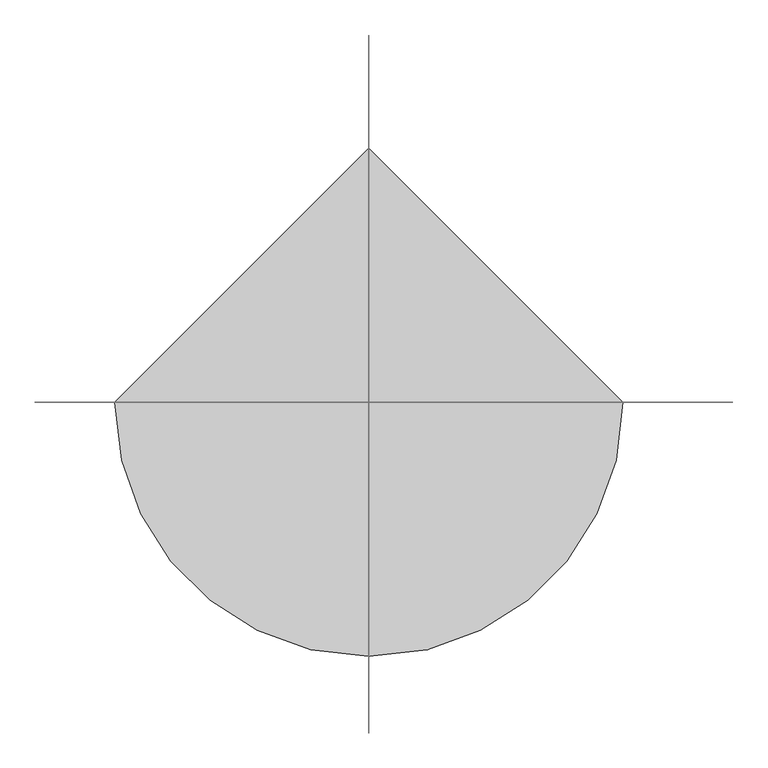
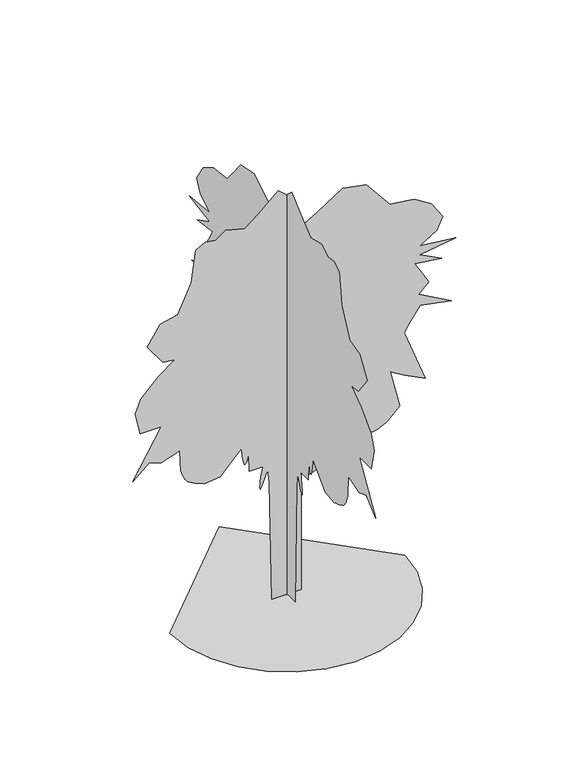
"""IFC4 building model written with IfcOpenShell, lengths in millimetres: proxy geometry, windmill palm 26123 : windmill palm 26123."""

from ifc_helpers import new_model, si_unit, origin, place, context, project, spatial, triangles, source, transform, mapped, element, save


def entourage_d7a905c7(model_context):
    return source(origin(), model_context, "Body", "Tessellation", [
        triangles([(-0.2241189, -80.6803134, 0.0560704), (-0.2241181, -93.4507094, 708.3955685), (-0.2241176, -102.9729479, 784.5729681), (-0.2241171, -112.4304103, 759.6428038), (-0.2241163, -121.4992608, 736.1299221), (-0.2241158, -129.7908604, 715.4466642), (-0.2241156, -136.916343, 699.0127836), (-0.2241151, -142.4870876, 688.2406214), (-0.2241151, -146.1147278, 684.5474602), (-0.2241148, -147.4101338, 689.3505827), (-0.2241148, -146.9475984, 700.5392893), (-0.2241151, -145.6519381, 714.7252693), (-0.2241151, -143.662352, 731.4105881), (-0.2241153, -141.1175219, 750.0923693), (-0.2241156, -138.1563745, 770.2752216), (-0.2241156, -134.9173553, 791.458885), (-0.2241158, -131.5396545, 813.1404104), (-0.2241113, -207.7180624, 813.1404104), (-0.224111, -210.8920511, 914.7103008), (-0.2241108, -214.9636775, 900.580204), (-0.2241105, -218.9799477, 887.367057), (-0.2241105, -222.88496, 875.9827955), (-0.2241103, -226.6235945, 867.3493109), (-0.22411, -230.1402221, 862.3810095), (-0.2241097, -233.3789961, 861.9923704), (-0.2241095, -236.2847599, 867.1003435), (-0.2241095, -238.9129061, 876.4653969), (-0.2241092, -241.3744383, 887.9944897), (-0.2241092, -243.6972616, 901.3295042), (-0.224109, -245.9088635, 916.1097794), (-0.224109, -248.0373855, 931.9696398), (-0.2241087, -250.1102786, 948.5533659), (-0.2241087, -252.1552483, 965.4977531), (-0.2241016, -372.7715778, 838.5329012), (-0.2240963, -461.6464946, 829.010372), (-0.224095, -479.2563572, 835.8125004), (-0.224094, -496.4217339, 842.6147015), (-0.2240932, -512.6981023, 849.4168299), (-0.2240922, -527.64352, 856.2164148), (-0.2240914, -540.8134646, 863.0185432), (-0.2240907, -551.7608706, 869.8206717), (-0.2240902, -560.0413244, 876.6228727), (-0.2240899, -566.4726179, 884.1641275), (-0.2240897, -572.238436, 893.0389492), (-0.2240892, -577.4480018, 903.0236595), (-0.2240889, -582.2155887, 913.8974871), (-0.2240887, -586.6479126, 925.4367537), (-0.2240884, -590.8567037, 937.4204699), (-0.2240881, -594.9562717, 949.6252481), (-0.2240879, -601.3062839, 1073.4150759), (-0.2240815, -706.0511621, 1038.5001286), (-0.2240775, -775.8810568, 1063.8925467), (-0.2240719, -867.928418, 981.3677147), (-0.2240815, -706.0511621, 1254.3398609), (-0.2240744, -826.6659657, 1254.3398609), (-0.2240727, -855.233408, 1381.3021694), (-0.2240747, -823.4909414, 1460.6545933), (-0.2240805, -725.0961479, 1562.224411), (-0.2240861, -629.8712191, 1632.0567764), (-0.2240821, -699.7011137, 1641.5768349), (-0.224077, -785.4035133, 1759.0190849), (-0.2240813, -712.3985945, 1873.2865288), (-0.2240871, -614.0012575, 1895.5039227), (-0.2240917, -537.8238579, 2060.5586735), (-0.2240932, -512.4314034, 2247.8284927), (-0.2240963, -458.4714704, 2276.3959351), (-0.2240998, -398.1640686, 2266.8734058), (-0.2241034, -341.0291113, 2308.1358582), (-0.2241097, -233.1107712, 2279.5708866), (-0.2241143, -156.9326267, 2339.8783974), (-0.2241212, -42.6652782, 2438.2757343), (-0.2241265, 46.2093524, 2358.9233105), (-0.2241265, 46.2093524, 2263.6984543), (-0.2241298, 103.3427746, 2190.6960789), (-0.2241346, 182.6954255, 2235.1334827), (-0.224143, 322.3549604, 2327.1809166), (-0.2241509, 455.6672811, 2301.7884258), (-0.2241557, 538.1921494, 2200.2186081), (-0.2241588, 588.979638, 2136.7361458), (-0.2241672, 728.6394636, 2117.6910873), (-0.224173, 827.0368006, 2057.3837219), (-0.2241768, 890.5167194, 1958.986385), (-0.2241748, 855.6017721, 1889.1564903), (-0.2241689, 760.3793867, 1828.8489796), (-0.2241811, 963.5216383, 1806.6315857), (-0.2241689, 760.3793867, 1774.8890465), (-0.2241763, 884.1692144, 1711.4067295), (-0.2241674, 731.8118717, 1730.4516426), (-0.224172, 811.1642956, 1593.9668049), (-0.2241687, 754.0318817, 1540.0068718), (-0.2241796, 938.1291475, 1435.2621025), (-0.2241692, 763.5544109, 1470.1769772), (-0.2241654, 700.0719486, 1384.477121), (-0.2241636, 671.5045063, 1336.8647655), (-0.224171, 792.1193098, 1022.630167), (-0.2241639, 674.6795305, 1079.7650517), (-0.224159, 592.1520824, 1130.5500332), (-0.2241621, 646.1120155, 908.3627958), (-0.2241583, 579.4571451, 841.7079254), (-0.2241575, 566.5462689, 834.2758209), (-0.2241567, 553.721761, 827.1511105), (-0.224156, 541.0623593, 820.6359558), (-0.2241552, 528.6518887, 815.0378237), (-0.2241544, 516.5766809, 810.6613466), (-0.2241537, 504.9155105, 807.8089771), (-0.2241532, 493.7572526, 806.7929054), (-0.2241524, 482.6879065, 807.6260668), (-0.2241519, 471.2883479, 809.9577559), (-0.2241511, 459.6093733, 813.5392233), (-0.2241504, 447.7094456, 818.1188129), (-0.2241496, 435.6418682, 823.4503189), (-0.2241489, 423.4625244, 829.2796143), (-0.2241481, 411.2298409, 835.357877), (-0.2241481, 407.7779803, 839.4116993), (-0.2241478, 404.0213056, 843.2979446), (-0.2241476, 399.6524952, 846.8514341), (-0.2241471, 394.3692784, 849.9070616), (-0.2241468, 387.8643339, 852.2946339), (-0.2241463, 379.8302676, 853.8491175), (-0.2241458, 369.9674249, 854.4028627), (-0.224145, 357.1403735, 855.883659), (-0.224144, 340.8157522, 860.0289728), (-0.2241428, 321.5777186, 866.3967527), (-0.2241415, 300.0079778, 874.5400057), (-0.2241402, 276.6881621, 884.0168255), (-0.2241387, 252.2014664, 894.3800737), (-0.2241372, 227.1326114, 905.1877716), (-0.2241349, 185.8694142, 857.577887), (-0.2241349, 185.8694142, 778.2254631), (-0.2241362, 208.0876256, 702.0480635), (-0.2241316, 131.9097354, 676.6556454), (-0.2241288, 87.4725496, 800.4429296), (-0.2241293, 88.096376, 0.0), (-666.8181644, -2.5e-06, 0.2128606), (-649.2007078, -152.6793797, 0.2128611), (-599.0329851, -292.8908795, 0.2128626), (-520.3257617, -416.61723, 0.2128649), (-417.1023385, -519.8431603, 0.2128679), (-293.3760243, -598.5478403, 0.2128717), (-153.1642702, -648.715563, 0.2128758), (-0.4850755, -666.3330196, 0.2128804), (152.1942349, -648.715563, 0.2128849), (292.4057347, -598.5478403, 0.212889), (416.1320852, -519.8406169, 0.2128928), (519.3580155, -416.61723, 0.2128959), (598.0626955, -292.8908795, 0.2128981), (648.2304182, -152.6791254, 0.2128997), (665.8478748, 5.82e-05, 0.2129002), (-0.4851924, 666.3330196, 0.2128804), (-89.341994, 0.0001455, 0.1894216), (-102.11239, 0.0001057, 708.5276825), (-111.6346285, 9.96e-05, 784.7075529), (-121.0920909, 0.0001025, 759.7773886), (-130.1609414, 0.0001023, 736.2619635), (-138.4522867, 0.0001051, 715.581249), (-145.5777693, 0.000105, 699.144825), (-151.1487682, 0.0001048, 688.3726627), (-154.7761631, 0.0001075, 684.682045), (-156.0718144, 0.0001043, 689.4852402), (-155.6090338, 0.0001041, 700.6714033), (-154.3136187, 0.0001037, 714.8573833), (-152.3240326, 0.0001034, 731.5426294), (-149.7792025, 0.0001031, 750.2269541), (-146.8178008, 9.98e-05, 770.4098791), (-143.5790359, 9.95e-05, 791.590999), (-140.2013351, 9.92e-05, 813.2725245), (-216.3794887, 9.82e-05, 813.2725245), (-219.5534773, 9.2e-05, 914.8448856), (-223.6253582, 9.2e-05, 900.7147888), (-227.6413739, 9.5e-05, 887.4991711), (-231.5466406, 9.5e-05, 876.1173803), (-235.2852751, 9.49e-05, 867.4838957), (-238.8016665, 9.47e-05, 862.5131235), (-242.0406767, 9.44e-05, 862.1244844), (-244.9461861, 9.4e-05, 867.2324575), (-247.5745867, 9.35e-05, 876.5974382), (-250.0361189, 9.29e-05, 888.1290745), (-252.358706, 9.23e-05, 901.464089), (-254.5697811, 9.17e-05, 916.2418934), (-256.6983031, 9.1e-05, 932.1042246), (-258.7709418, 9.04e-05, 948.6854073), (-260.8156571, 8.97e-05, 965.6297945), (-381.4330041, 9.73e-05, 838.667486), (-470.3079208, 9.84e-05, 829.1450294), (-487.9177835, 9.66e-05, 835.9446144), (-505.0831601, 9.78e-05, 842.7467428), (-521.3595285, 9.61e-05, 849.5488712), (-536.3049462, 9.46e-05, 856.3510723), (-549.4748909, 9.61e-05, 863.1532007), (-560.4222968, 9.49e-05, 869.9527857), (-568.7027507, 9.4e-05, 876.7549141), (-575.1340442, 9.32e-05, 884.2962416), (-580.8998623, 9.24e-05, 893.1709906), (-586.109428, 9.17e-05, 903.1557735), (-590.8770149, 9.38e-05, 914.0295284), (-595.3093389, 9.31e-05, 925.568795), (-599.5181299, 9.23e-05, 937.5525839), (-603.617698, 9.16e-05, 949.759833), (-609.9677101, 8.15e-05, 1073.5496607), (-714.7125521, 8.49e-05, 1038.6347134), (-784.5424467, 8.37e-05, 1064.0272041), (-876.5898079, 8.96e-05, 981.4997561), (-714.7125521, 7.26e-05, 1254.4719749), (-835.3274282, 7.35e-05, 1254.4719749), (-863.8948706, 6.42e-05, 1381.4367542), (-832.152404, 5.89e-05, 1460.7891781), (-733.7575378, 5.3e-05, 1562.3589958), (-638.532609, 5.06e-05, 1632.1888905), (-708.3625763, 4.99e-05, 1641.7114197), (-794.0649759, 4.17e-05, 1759.1538151), (-721.0600571, 3.61e-05, 1873.4184975), (-622.6626474, 3.25e-05, 1895.6385075), (-546.4852841, 2.27e-05, 2060.6907875), (-521.0928297, 1.36e-05, 2247.9630775), (-467.1328966, 1.17e-05, 2276.5305199), (-406.8254949, 1.15e-05, 2267.0079906), (-349.6905375, 9.6e-06, 2308.270443), (-241.7724518, 1.13e-05, 2279.7030006), (-165.5940529, 7.6e-06, 2340.0103661), (-51.3267045, 3e-07, 2438.4078484), (37.5476695, 7.7e-06, 2359.0554245), (37.5476695, 1.34e-05, 2263.8330391), (94.6810849, 1.78e-05, 2190.8281929), (174.0337449, 1.48e-05, 2235.2655968), (313.6935342, 7e-06, 2327.3155014), (447.0058548, 1.09e-05, 2301.9230106), (529.5307231, 1.55e-05, 2200.3505768), (580.3182117, 1.9e-05, 2136.8682598), (719.978001, 2.04e-05, 2117.8258175), (818.3728672, 2.51e-05, 2057.515836), (881.8552568, 3.08e-05, 1959.1209698), (846.9403095, 3.56e-05, 1889.2910751), (751.7179241, 3.77e-05, 1828.9837097), (954.8601757, 3.9e-05, 1806.7636997), (751.7179241, 4.22e-05, 1775.0237766), (875.5077518, 4.35e-05, 1711.5413143), (723.1504818, 4.39e-05, 1730.5862274), (802.502833, 5.21e-05, 1594.0989189), (745.3704918, 5.45e-05, 1540.1416019), (929.4676849, 6.24e-05, 1435.3942165), (754.8929483, 6.03e-05, 1470.3117073), (691.4105587, 6.3e-05, 1384.609235), (662.8430437, 6.77e-05, 1336.9993504), (783.4579199, 8.5e-05, 1022.7647518), (666.0180679, 8.15e-05, 1079.8971657), (583.4906562, 7.85e-05, 1130.6820745), (637.4506256, 9.28e-05, 908.4973806), (570.7957189, 9.76e-05, 841.8399668), (557.8848427, 9.67e-05, 834.4104784), (545.0603348, 9.87e-05, 827.2831518), (532.4009331, 9.77e-05, 820.7706133), (519.9904624, 9.97e-05, 815.169865), (507.9152547, 9.88e-05, 810.7934607), (496.2540842, 9.78e-05, 807.9435619), (485.0932829, 9.98e-05, 806.9250195), (474.0264802, 9.87e-05, 807.7581808), (462.6269217, 9.77e-05, 810.0898699), (450.947947, 9.94e-05, 813.6712646), (439.0480193, 9.82e-05, 818.2534704), (426.980442, 9.7e-05, 823.5823603), (414.8010982, 9.86e-05, 829.4117283), (402.5684146, 9.74e-05, 835.4924618), (399.1165541, 9.69e-05, 839.5463568), (395.3598793, 9.65e-05, 843.4325294), (390.9910689, 9.6e-05, 846.9860189), (385.7078522, 9.54e-05, 850.0391029), (379.2029077, 9.48e-05, 852.4267479), (371.1688414, 9.69e-05, 853.9812315), (361.3059986, 9.6e-05, 854.5374475), (348.4789473, 9.48e-05, 856.0183165), (332.154326, 9.62e-05, 860.1635576), (312.9162924, 9.43e-05, 866.5288668), (291.3465516, 9.5e-05, 874.6721197), (268.0267359, 9.56e-05, 884.1488668), (243.5397858, 9.31e-05, 894.5146585), (218.4709308, 9.34e-05, 905.3224291), (177.2077336, 9.7e-05, 857.7099283), (177.2077336, 9.94e-05, 778.3575771), (199.4261993, 0.0001036, 702.1801775), (123.2483092, 0.0001063, 676.7876867), (78.8108599, 9.87e-05, 800.5775145), (79.4346863, 0.0001459, 0.1333563)], [[85, 84, 86], [53, 52, 54], [91, 90, 92], [87, 86, 88], [95, 94, 96], [96, 94, 97], [9, 8, 10], [52, 51, 54], [51, 50, 54], [1, 133, 2], [133, 132, 2], [2, 132, 3], [131, 130, 132], [130, 129, 132], [129, 128, 132], [18, 17, 19], [71, 70, 72], [72, 70, 73], [10, 8, 11], [8, 7, 11], [11, 7, 12], [7, 6, 12], [12, 6, 13], [6, 5, 13], [13, 5, 14], [5, 4, 14], [14, 4, 15], [4, 3, 15], [15, 3, 16], [16, 3, 17], [55, 54, 56], [89, 88, 90], [56, 54, 57], [57, 54, 58], [61, 60, 62], [62, 60, 63], [60, 59, 63], [25, 24, 26], [24, 23, 26], [26, 23, 27], [23, 22, 27], [27, 22, 28], [22, 21, 28], [28, 21, 29], [21, 20, 29], [29, 20, 30], [20, 19, 30], [30, 19, 31], [82, 81, 83], [83, 81, 84], [81, 80, 84], [80, 79, 84], [70, 69, 73], [98, 97, 99], [31, 19, 32], [99, 97, 100], [58, 54, 59], [100, 97, 101], [101, 97, 102], [102, 97, 103], [103, 97, 104], [104, 97, 105], [105, 97, 106], [106, 97, 107], [107, 97, 108], [108, 97, 109], [109, 97, 110], [110, 97, 111], [111, 97, 112], [112, 97, 113], [113, 97, 114], [114, 97, 115], [115, 97, 116], [116, 97, 117], [117, 97, 118], [118, 97, 119], [119, 97, 120], [120, 97, 121], [121, 97, 122], [122, 97, 123], [123, 97, 124], [124, 97, 125], [125, 97, 126], [126, 97, 127], [65, 64, 66], [66, 64, 67], [68, 67, 69], [67, 64, 69], [3, 132, 17], [73, 69, 74], [69, 64, 74], [64, 63, 74], [63, 59, 74], [17, 132, 19], [132, 128, 19], [128, 127, 19], [92, 90, 93], [76, 75, 77], [77, 75, 78], [78, 75, 79], [79, 75, 84], [75, 74, 84], [74, 59, 84], [84, 59, 86], [86, 59, 88], [88, 59, 90], [90, 59, 93], [93, 59, 94], [94, 59, 97], [97, 59, 127], [127, 59, 19], [32, 19, 33], [19, 59, 33], [59, 54, 33], [54, 50, 33], [33, 50, 34], [50, 49, 34], [34, 49, 35], [35, 49, 36], [36, 49, 37], [49, 48, 37], [37, 48, 38], [48, 47, 38], [38, 47, 39], [47, 46, 39], [39, 46, 40], [46, 45, 40], [45, 44, 40], [40, 44, 41], [44, 43, 41], [41, 43, 42], [148, 149, 134], [147, 148, 134], [147, 134, 135], [146, 147, 135], [146, 135, 136], [146, 136, 137], [145, 146, 137], [144, 145, 137], [144, 137, 138], [144, 138, 139], [144, 139, 140], [144, 140, 141], [144, 141, 142], [144, 142, 143], [233, 234, 235], [201, 202, 203], [239, 240, 241], [235, 236, 237], [243, 244, 245], [243, 245, 246], [157, 158, 159], [200, 201, 203], [199, 200, 203], [282, 150, 151], [281, 282, 151], [281, 151, 152], [279, 280, 281], [278, 279, 281], [277, 278, 281], [166, 167, 168], [219, 220, 221], [219, 221, 222], [157, 159, 160], [156, 157, 160], [156, 160, 161], [155, 156, 161], [155, 161, 162], [154, 155, 162], [154, 162, 163], [153, 154, 163], [153, 163, 164], [152, 153, 164], [152, 164, 165], [152, 165, 166], [203, 204, 205], [237, 238, 239], [203, 205, 206], [203, 206, 207], [209, 210, 211], [209, 211, 212], [208, 209, 212], [173, 174, 175], [172, 173, 175], [172, 175, 176], [171, 172, 176], [171, 176, 177], [170, 171, 177], [170, 177, 178], [169, 170, 178], [169, 178, 179], [168, 169, 179], [168, 179, 180], [230, 231, 232], [230, 232, 233], [229, 230, 233], [228, 229, 233], [218, 219, 222], [246, 247, 248], [168, 180, 181], [246, 248, 249], [203, 207, 208], [246, 249, 250], [246, 250, 251], [246, 251, 252], [246, 252, 253], [246, 253, 254], [246, 254, 255], [246, 255, 256], [246, 256, 257], [246, 257, 258], [246, 258, 259], [246, 259, 260], [246, 260, 261], [246, 261, 262], [246, 262, 263], [246, 263, 264], [246, 264, 265], [246, 265, 266], [246, 266, 267], [246, 267, 268], [246, 268, 269], [246, 269, 270], [246, 270, 271], [246, 271, 272], [246, 272, 273], [246, 273, 274], [246, 274, 275], [246, 275, 276], [213, 214, 215], [213, 215, 216], [216, 217, 218], [213, 216, 218], [281, 152, 166], [218, 222, 223], [213, 218, 223], [212, 213, 223], [208, 212, 223], [281, 166, 168], [277, 281, 168], [276, 277, 168], [239, 241, 242], [224, 225, 226], [224, 226, 227], [224, 227, 228], [224, 228, 233], [223, 224, 233], [208, 223, 233], [208, 233, 235], [208, 235, 237], [208, 237, 239], [208, 239, 242], [208, 242, 243], [208, 243, 246], [208, 246, 276], [208, 276, 168], [168, 181, 182], [208, 168, 182], [203, 208, 182], [199, 203, 182], [199, 182, 183], [198, 199, 183], [198, 183, 184], [198, 184, 185], [198, 185, 186], [197, 198, 186], [197, 186, 187], [196, 197, 187], [196, 187, 188], [195, 196, 188], [195, 188, 189], [194, 195, 189], [193, 194, 189], [193, 189, 190], [192, 193, 190], [192, 190, 191]], closed=False),
    ])


if __name__ == "__main__":
    model = new_model("IFC4")
    model_context = context("Model", 3, world=origin())
    ifc_project = project(units=[si_unit("LENGTHUNIT", "METRE", prefix="MILLI")], contexts=[model_context])
    site = spatial("IfcSite", under=ifc_project)
    building = spatial("IfcBuilding", under=site)
    placement = place(None, origin())
    entourage_shape = entourage_d7a905c7(model_context)
    element("IfcBuildingElementProxy", 1, Name="windmill palm 26123 : windmill palm 26123", ObjectType="windmill palm 26123 : windmill palm 26123", at=placement, inside=building, context=model_context, shape_type="MappedRepresentation", body=[
        mapped(entourage_shape, transform((0.0, 0.0, 0.0), x_axis=(1.0, 0.0, 0.0), y_axis=(0.0, 1.0, 0.0), z_axis=(0.0, 0.0, 1.0))),
    ])
    save(model, "model.ifc")

# Revit data of these elements
# Type "windmill palm 26123 : windmill palm 26123"
#   built-in parameter 1005195 = "RPC-16-G2MF-J1Q0-CAN1-N000-ST1L-LVER-AU"
#   Height = 0
